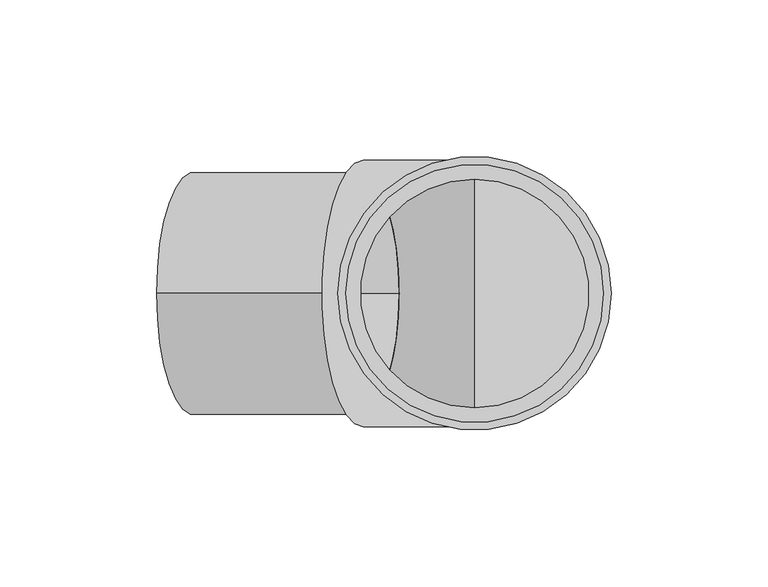
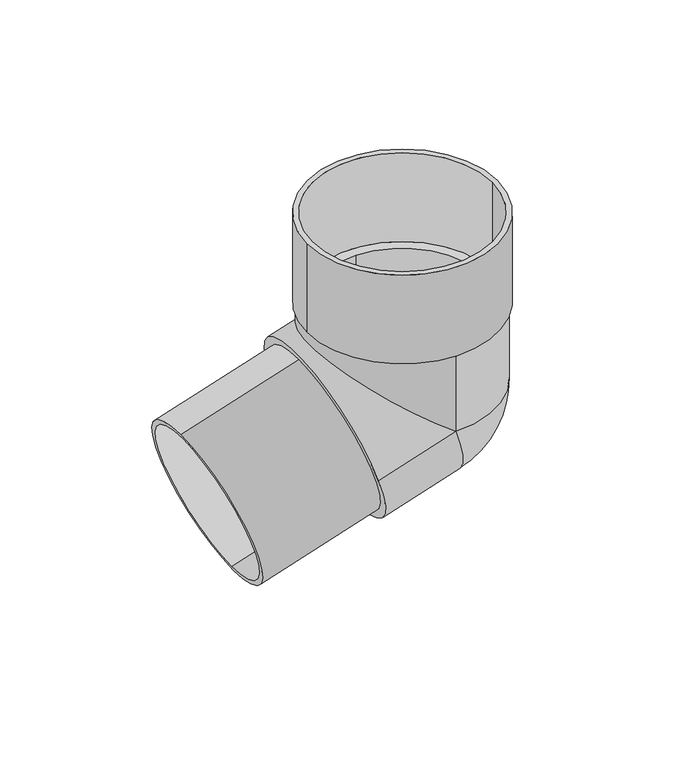
"""IFC4 building model written with IfcOpenShell, lengths in millimetres: proxy geometry, ⇲ Колено трубы 108 : ⇲ Колено трубы 108."""

from ifc_helpers import new_model, si_unit, point, frame, origin, origin_with_axes, origin_2d, place, context, project, spatial, polyline, circle_curve, ellipse_curve, trimmed, segment, composite_curve, outline, extrude, source, transform, mapped, element, save
from ifc_brep_helpers import plane_surface, cylinder_surface, revolved_surface, advanced_brep


def generic_models_e50198c4(model_context):
    return source(origin(), model_context, "Body", "SolidModel", [
        extrude(outline(composite_curve([segment(trimmed(circle_curve(origin_2d(), 38.8), [point((0.0, 38.8))], [point((0.0, -38.8000001))], False, "CARTESIAN"), True, "CONTINUOUS"), segment(trimmed(circle_curve(origin_2d(), 38.8), [point((0.0, -38.8000001))], [point((0.0, 38.8))], False, "CARTESIAN"), True, "CONTINUOUS")], self_intersect=False), holes=[composite_curve([segment(trimmed(circle_curve(origin_2d(), 36.5), [point((0.0, 36.5))], [point((0.0, -36.5000001))], True, "CARTESIAN"), True, "CONTINUOUS"), segment(trimmed(circle_curve(origin_2d(), 36.5), [point((0.0, -36.5000001))], [point((0.0, 36.5))], True, "CARTESIAN"), True, "CONTINUOUS")], self_intersect=False)]), frame((-89.3993125, 0.0, -109.2975975), z_axis=(0.9510565162951546, 0.0, 0.30901699437494445), x_axis=(0.0, -1.0, 0.0)), (0.0, 0.0, 1.0), 56.7),
        advanced_brep(
        [(41.1, 0.0, -43.0), (-41.1, 0.0, -43.0), (0.0, 36.41, -43.0), (0.0, -36.41, -43.0), (0.0, 42.5, -43.0), (0.0, 42.5, -80.25), (0.0, -42.5, -80.25), (0.0, -42.5, -43.0), (42.5, 0.0, -80.25), (0.0, 36.41, -80.25), (0.0, -36.41, -80.25), (-35.4744081, 42.5, -91.7763339), (-35.4744081, -42.5, -91.7763339), (-35.4744081, 36.41, -91.7763339), (-35.4744081, -36.41, -91.7763339), (13.1332223, 0.0, -120.6699019), (-43.6, 0.0, 0.0), (43.6, 0.0, 0.0), (-41.1, 0.0, 0.0), (41.1, 0.0, 0.0), (-43.6, 0.0, -43.0), (43.6, 0.0, -43.0)],
        [
            (0, 1, circle_curve(frame((0.0, 0.0, -43.0), z_axis=(0.0, 0.0, 1.0), x_axis=(1.0, 0.0, 0.0)), 41.1)),
            (1, 0, circle_curve(frame((0.0, 0.0, -43.0), z_axis=(0.0, 0.0, 1.0), x_axis=(1.0, 0.0, 0.0)), 41.1)),
            (2, 3, circle_curve(frame((0.0, 0.0, -43.0), z_axis=(0.0, 0.0, -1.0), x_axis=(0.0, -1.0, 0.0)), 36.41)),
            (3, 2, circle_curve(frame((0.0, 0.0, -43.0), z_axis=(0.0, 0.0, -1.0), x_axis=(0.0, -1.0, 0.0)), 36.41)),
            (4, 5),
            (5, 6, ellipse_curve(frame((0.0, 0.0, -80.25), z_axis=(0.5877852522924751, 0.0, 0.8090169943749459), x_axis=(-0.8090169943749458, 0.0, 0.5877852522924751)), 52.532889, 42.5)),
            (6, 7),
            (7, 4, circle_curve(frame((0.0, 0.0, -43.0), z_axis=(0.0, 0.0, -1.0), x_axis=(0.0, -1.0, 0.0)), 42.5)),
            (4, 7, circle_curve(frame((0.0, 0.0, -43.0), z_axis=(0.0, 0.0, -1.0), x_axis=(0.0, -1.0, 0.0)), 42.5)),
            (6, 8, circle_curve(frame((0.0, 0.0, -80.25), z_axis=(0.0, 0.0, 1.0), x_axis=(0.0, -1.0, 0.0)), 42.5)),
            (8, 5, circle_curve(frame((0.0, 0.0, -80.25), z_axis=(0.0, 0.0, 1.0), x_axis=(0.0, -1.0, 0.0)), 42.5)),
            (2, 9),
            (9, 10, circle_curve(frame((0.0, 0.0, -80.25), z_axis=(0.0, 0.0, -1.0), x_axis=(0.0, -1.0, 0.0)), 36.41)),
            (10, 3),
            (10, 9, ellipse_curve(frame((0.0, 0.0, -80.25), z_axis=(-0.5877852522924751, 0.0, -0.8090169943749459), x_axis=(0.8090169943749458, 0.0, -0.5877852522924751)), 45.0052351, 36.41)),
            (11, 12, circle_curve(frame((-35.4744081, 0.0, -91.7763339), z_axis=(-0.9510565162951546, 0.0, -0.30901699437494445), x_axis=(0.0, -1.0, 0.0)), 42.5)),
            (12, 11, circle_curve(frame((-35.4744081, 0.0, -91.7763339), z_axis=(-0.9510565162951546, 0.0, -0.30901699437494445), x_axis=(0.0, -1.0, 0.0)), 42.5)),
            (13, 14, circle_curve(frame((-35.4744081, 0.0, -91.7763339), z_axis=(0.9510565162951546, 0.0, 0.30901699437494445), x_axis=(0.0, -1.0, 0.0)), 36.41)),
            (14, 13, circle_curve(frame((-35.4744081, 0.0, -91.7763339), z_axis=(0.9510565162951546, 0.0, 0.30901699437494445), x_axis=(0.0, -1.0, 0.0)), 36.41)),
            (5, 11),
            (12, 6),
            (5, 15, circle_curve(frame((0.0, 0.0, -80.25), z_axis=(-0.9510565162951546, 0.0, -0.30901699437494445), x_axis=(0.0, -1.0, 0.0)), 42.5)),
            (15, 6, circle_curve(frame((0.0, 0.0, -80.25), z_axis=(-0.9510565162951546, 0.0, -0.30901699437494445), x_axis=(0.0, -1.0, 0.0)), 42.5)),
            (14, 10),
            (10, 9, circle_curve(frame((0.0, 0.0, -80.25), z_axis=(0.9510565162951546, 0.0, 0.30901699437494445), x_axis=(0.0, -1.0, 0.0)), 36.41)),
            (9, 13),
            (9, 10),
            (16, 17, circle_curve(origin_with_axes(), 43.6)),
            (17, 16, circle_curve(origin_with_axes(), 43.6)),
            (18, 19, circle_curve(frame((0.0, 0.0, 0.0), z_axis=(0.0, 0.0, -1.0), x_axis=(1.0, 0.0, 0.0)), 41.1)),
            (19, 18, circle_curve(frame((0.0, 0.0, 0.0), z_axis=(0.0, 0.0, -1.0), x_axis=(1.0, 0.0, 0.0)), 41.1)),
            (20, 21, circle_curve(frame((0.0, 0.0, -43.0), z_axis=(0.0, 0.0, -1.0), x_axis=(1.0, 0.0, 0.0)), 43.6)),
            (21, 20, circle_curve(frame((0.0, 0.0, -43.0), z_axis=(0.0, 0.0, -1.0), x_axis=(1.0, 0.0, 0.0)), 43.6)),
            (18, 1),
            (0, 19),
            (16, 20),
            (21, 17),
        ],
        [
            plane_surface(frame((0.0, 0.0, -43.0), z_axis=(0.0, 0.0, 1.0), x_axis=(0.0, -1.0, 0.0))),
            cylinder_surface(frame((0.0, 0.0, -43.0), z_axis=(0.0, 0.0, 1.0), x_axis=(0.0, -1.0, 0.0)), 42.5),
            revolved_surface(polyline([(0.0, -36.41, -80.25), (0.0, -36.41, -43.0)]), (0.0, 0.0, -43.0), (0.0, 0.0, -1.0)),
            revolved_surface(polyline([(0.0, -36.41, -106.70341346773566), (0.0, -36.41, -43.0)]), (0.0, 0.0, -43.0), (0.0, 0.0, -1.0)),
            plane_surface(frame((-35.4744081, 0.0, -91.7763339), z_axis=(-0.9510565162951546, 0.0, -0.30901699437494445), x_axis=(0.0, -1.0, 0.0))),
            cylinder_surface(frame((0.0, 0.0, -80.25), z_axis=(0.9510565162951546, 0.0, 0.30901699437494445), x_axis=(0.0, -1.0, 0.0)), 42.5),
            revolved_surface(polyline([(-35.47440809885558, -36.41, -91.77633390352219), (0.0, -36.41, -80.25)]), (0.0, 0.0, -80.25), (-0.9510565162951546, 0.0, -0.30901699437494445)),
            revolved_surface(polyline([(-35.47440809885558, -36.41, -91.77633390352219), (25.15869125673993, -36.41, -72.07544567924268)]), (0.0, 0.0, -80.25), (-0.9510565162951546, 0.0, -0.30901699437494445)),
            plane_surface(frame((0.0, 50.0, -80.25), z_axis=(0.0, 0.0, 1.0), x_axis=(1.0, 0.0, 0.0))),
            plane_surface(frame((0.0, 50.0, -80.25), z_axis=(-0.9510565162951546, 0.0, -0.30901699437494445), x_axis=(0.30901699437494445, 0.0, -0.9510565162951546))),
            revolved_surface(trimmed(ellipse_curve(frame((0.0, 0.0, -80.25), z_axis=(0.0, 0.0, 1.0), x_axis=(1.0, 0.0, 0.0)), 42.5, 42.5), [point((0.0, -42.5, -80.25))], [point((0.0, 42.5, -80.25))], True, "CARTESIAN"), (0.0, 50.0, -80.25), (0.0, 1.0, 0.0)),
            plane_surface(frame((41.1, 0.0, 0.0), z_axis=(0.0, 0.0, 1.0), x_axis=(0.0, -1.0, 0.0))),
            plane_surface(frame((41.1, 0.0, -43.0), z_axis=(0.0, 0.0, -1.0), x_axis=(0.0, 1.0, 0.0))),
            revolved_surface(polyline([(41.1, 0.0, -43.0), (41.1, 0.0, 0.0)]), (0.0, 0.0, -43.0), (0.0, 0.0, -1.0)),
            cylinder_surface(origin_with_axes(), 43.6),
        ],
        [
            (0, [[1, 2], [3, 4]]),
            (1, [[5, 6, 7, 8]]),
            (1, [[-5, 9, -7, 10, 11]]),
            (2, [[-3, 12, 13, 14]]),
            (3, [[-4, -14, 15, -12]]),
            (4, [[16, 17], [18, 19]]),
            (5, [[-6, 20, -17, 21]]),
            (5, [[-16, -20, 22, 23, -21]]),
            (6, [[-19, 24, 25, 26]]),
            (7, [[-15, -24, -18, -26]]),
            (8, [[27, -13]]),
            (9, [[-27, -25]]),
            (10, [[-11, -10, -23, -22]]),
            (11, [[28, 29], [30, 31]]),
            (12, [[32, 33], [-8, -9]]),
            (13, [[-30, 34, -1, 35]]),
            (13, [[-31, -35, -2, -34]]),
            (14, [[-28, 36, -33, 37]]),
            (14, [[-29, -37, -32, -36]]),
        ],
    ),
    ])


if __name__ == "__main__":
    model = new_model("IFC4")
    model_context = context("Model", 3, world=origin())
    ifc_project = project(units=[si_unit("LENGTHUNIT", "METRE", prefix="MILLI")], contexts=[model_context])
    site = spatial("IfcSite", under=ifc_project)
    building = spatial("IfcBuilding", under=site)
    placement = place(None, origin())
    generic_models_shape = generic_models_e50198c4(model_context)
    element("IfcBuildingElementProxy", 1, Name="⇲ Колено трубы 108 : ⇲ Колено трубы 108", ObjectType="⇲ Колено трубы 108 : ⇲ Колено трубы 108", at=placement, inside=building, context=model_context, shape_type="MappedRepresentation", body=[
        mapped(generic_models_shape, transform((0.0, 0.0, 0.0), x_axis=(1.0, 0.0, 0.0), y_axis=(0.0, 1.0, 0.0), z_axis=(0.0, 0.0, 1.0))),
    ])
    save(model, "model.ifc")

# Revit data of these elements
# Type "⇲ Колено трубы 108 : ⇲ Колено трубы 108"
#   Description = "Предназначено для изменения направления стока по трубе. Также применяется для обхода архитектурных элементов\r\nфасада"
#   Manufacturer = "ТехноНИКОЛЬ"
#   Model = "Комплектующие к водосточным системам"
#   URL = "https://tn-vodostok.ru/catalog/pvh/"
#   ADSK_Обозначение = "ТехноНИКОЛЬ"
#   ADSK_Наименование краткое = "Колено 108°"
#   ADSK_Наименование = "Колено трубы 108°"
#   ADSK_Масса_Текст = ""
#   ADSK_Марка = ""
#   ADSK_Код изделия = ""
#   ADSK_Завод-изготовитель = "ТехноНИКОЛЬ"
#   ADSK_Единица измерения = "шт."
#   ADSK_Группирование = "Комплектующие к водосточным системам"
#   ADSK_URL страницы изделия = "https://tn-vodostok.ru/catalog/pvh/"
#   ADSK_URL документации изделия = "https://tn-vodostok.ru/upload/iblock/c42/c427963cb77eb5c3c51f0cfb870e9e52.pdf"
#   Угол поворота хомута [instance default] = 0.00°
#   ADSK_Размер_Ширина = 145.3 mm
#   ADSK_Размер_Диаметр = 82.2 mm
#   ADSK_Размер_Высота = 160.5 mm
#   ADSK_Количество = 1
#   ADSK_Материал [instance default] = TN_Пластик_Коричневый_RAL8019
#   Default Elevation = 0
# Element 1 (IfcBuildingElementProxy, "⇲ Колено трубы 108 : ⇲ Колено трубы 108")
#   Materials on its faces: "TN_Пластик_Коричневый_RAL8019"
# Materials
#   "TN_Пластик_Коричневый_RAL8019": class "Типовые", colour RGB 61 54 53, transparency 0, Cost = 0
